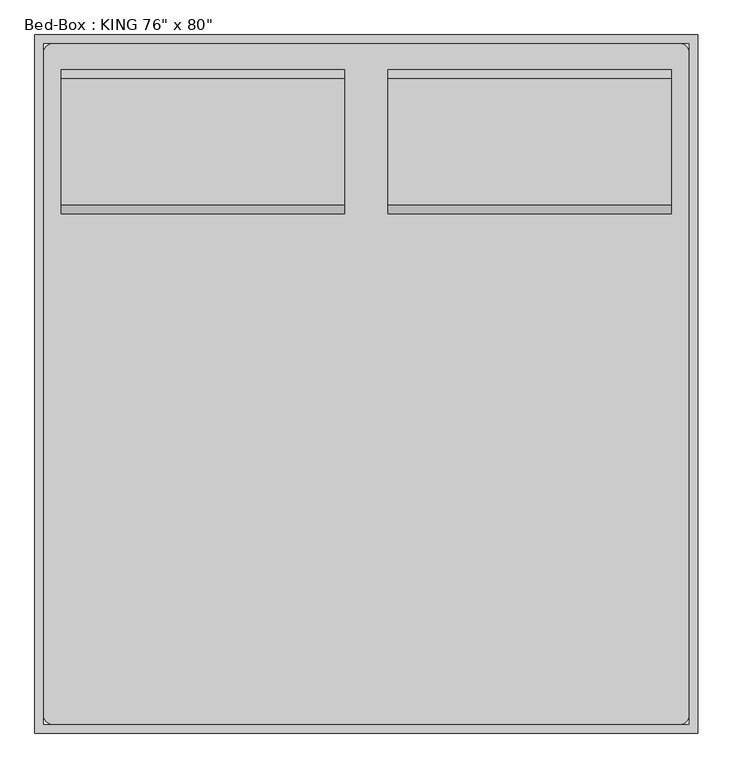
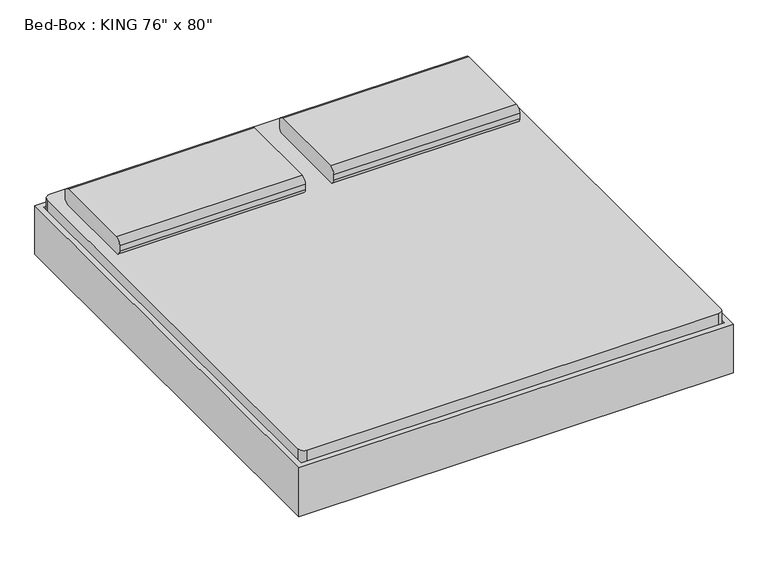
"""IFC4 building model written with IfcOpenShell, lengths in millimetres: furniture geometry."""

from ifc_helpers import new_model, si_unit, point, frame, frame_2d, origin, place, context, project, spatial, polyline, circle_curve, trimmed, segment, composite_curve, outline, extrude, source, transform, mapped, element, save
from ifc_brep_helpers import plane_surface, cylinder_surface, revolved_surface, advanced_brep


def furniture_3daafeb3(model_context):
    return source(origin(), model_context, "Body", "SolidModel", [
        extrude(outline(composite_curve([segment(polyline([(654.5704918, 406.4), (286.2704918, 406.4)]), True, "CONTINUOUS"), segment(trimmed(circle_curve(frame_2d((286.2704918, 431.8)), 25.4), [point((286.2704918, 406.4))], [point((260.8704918, 431.8))], False, "CARTESIAN"), True, "CONTINUOUS"), segment(polyline([(260.8704918, 431.8), (260.8704918, 457.2)]), True, "CONTINUOUS"), segment(trimmed(circle_curve(frame_2d((286.2704918, 457.2)), 25.4), [point((260.8704918, 457.2))], [point((286.2704918, 482.6))], False, "CARTESIAN"), True, "CONTINUOUS"), segment(polyline([(286.2704918, 482.6), (654.5704918, 482.6)]), True, "CONTINUOUS"), segment(trimmed(circle_curve(frame_2d((654.5704918, 457.2)), 25.4), [point((654.5704918, 482.6))], [point((679.9704918, 457.2))], False, "CARTESIAN"), True, "CONTINUOUS"), segment(polyline([(679.9704918, 457.2), (679.9704918, 431.8)]), True, "CONTINUOUS"), segment(trimmed(circle_curve(frame_2d((654.5704918, 431.8)), 25.4), [point((679.9704918, 431.8))], [point((654.5704918, 406.4))], False, "CARTESIAN"), True, "CONTINUOUS")], self_intersect=False)), frame((402.652459, 0.0, 0.0), z_axis=(1.0, 0.0, 0.0), x_axis=(0.0, 1.0, 0.0)), (0.0, 0.0, 1.0), 825.5),
        extrude(outline(composite_curve([segment(polyline([(654.5704918, 406.4), (286.2704918, 406.4)]), True, "CONTINUOUS"), segment(trimmed(circle_curve(frame_2d((286.2704918, 431.8)), 25.4), [point((286.2704918, 406.4))], [point((260.8704918, 431.8))], False, "CARTESIAN"), True, "CONTINUOUS"), segment(polyline([(260.8704918, 431.8), (260.8704918, 457.2)]), True, "CONTINUOUS"), segment(trimmed(circle_curve(frame_2d((286.2704918, 457.2)), 25.4), [point((260.8704918, 457.2))], [point((286.2704918, 482.6))], False, "CARTESIAN"), True, "CONTINUOUS"), segment(polyline([(286.2704918, 482.6), (654.5704918, 482.6)]), True, "CONTINUOUS"), segment(trimmed(circle_curve(frame_2d((654.5704918, 457.2)), 25.4), [point((654.5704918, 482.6))], [point((679.9704918, 457.2))], False, "CARTESIAN"), True, "CONTINUOUS"), segment(polyline([(679.9704918, 457.2), (679.9704918, 431.8)]), True, "CONTINUOUS"), segment(trimmed(circle_curve(frame_2d((654.5704918, 431.8)), 25.4), [point((679.9704918, 431.8))], [point((654.5704918, 406.4))], False, "CARTESIAN"), True, "CONTINUOUS")], self_intersect=False)), frame((-549.847541, 0.0, 0.0), z_axis=(1.0, 0.0, 0.0), x_axis=(0.0, 1.0, 0.0)), (0.0, 0.0, 1.0), 825.5),
        advanced_brep(
        [(-600.3231784, 527.5704918, 177.8), (-600.3231784, 451.3704918, 177.8), (-600.3231784, 451.3704918, 196.85), (-600.3231784, 527.5704918, 196.85), (-549.5231784, 527.5704918, 177.8), (-549.5231784, 451.3704918, 177.8), (-537.3869899, 451.3704918, 196.85), (-537.3869899, 527.5704918, 196.85), (-473.4523099, 527.5704918, 14.6654962), (-473.4523099, 451.3704918, 14.6654962), (-456.1871466, 451.3704918, 22.716374), (-456.1871466, 527.5704918, 22.716374), (-450.4320921, 451.3704918, 0.0), (-450.4320921, 527.5704918, 0.0), (-450.4320921, 451.3704918, 19.05), (-450.4320921, 527.5704918, 19.05), (-371.8195862, 527.5704918, 0.0), (-371.8195862, 451.3704918, 0.0), (-371.8195862, 451.3704918, 19.05), (-371.8195862, 527.5704918, 19.05), (-359.1195862, 451.3704918, 3.4029547), (-359.1195862, 527.5704918, 3.4029547), (-368.6445862, 451.3704918, 19.9007387), (-368.6445862, 527.5704918, 19.9007387), (-299.022541, 527.5704918, 38.1), (-299.022541, 451.3704918, 38.1), (-304.1269731, 451.3704918, 57.15), (-304.1269731, 527.5704918, 57.15), (977.6518216, 527.5704918, 38.1), (977.6518216, 451.3704918, 38.1), (982.7562537, 451.3704918, 57.15), (982.7562537, 527.5704918, 57.15), (1037.7488669, 527.5704918, 3.4029547), (1037.7488669, 451.3704918, 3.4029547), (1047.2738669, 451.3704918, 19.9007387), (1047.2738669, 527.5704918, 19.9007387), (1050.4488669, 451.3704918, 0.0), (1050.4488669, 527.5704918, 0.0), (1050.4488669, 451.3704918, 19.05), (1050.4488669, 527.5704918, 19.05), (1129.0613728, 527.5704918, 0.0), (1129.0613728, 451.3704918, 0.0), (1129.0613728, 451.3704918, 19.05), (1129.0613728, 527.5704918, 19.05), (1152.0815906, 451.3704918, 14.6654962), (1152.0815906, 527.5704918, 14.6654962), (1134.8164272, 451.3704918, 22.716374), (1134.8164272, 527.5704918, 22.716374), (1228.152459, 527.5704918, 177.8), (1228.152459, 451.3704918, 177.8), (1216.0162705, 451.3704918, 196.85), (1216.0162705, 527.5704918, 196.85), (1278.952459, 527.5704918, 177.8), (1278.952459, 527.5704918, 196.85), (1278.952459, 451.3704918, 196.85), (1278.952459, 451.3704918, 177.8)],
        [
            (0, 1),
            (1, 2),
            (2, 3),
            (3, 0),
            (0, 4),
            (4, 5),
            (5, 1),
            (5, 6),
            (6, 2),
            (6, 7),
            (7, 3),
            (7, 4),
            (4, 8),
            (8, 9),
            (9, 5),
            (9, 10),
            (10, 6),
            (10, 11),
            (11, 7),
            (11, 8),
            (12, 9, circle_curve(frame((-450.4320921, 451.3704918, 25.4), z_axis=(0.0, 1.0, 0.0), x_axis=(-0.9063077870366486, 0.0, -0.42261826174070233)), 25.4)),
            (8, 13, circle_curve(frame((-450.4320921, 527.5704918, 25.4), z_axis=(0.0, -1.0, 0.0), x_axis=(-0.9063077870366486, 0.0, -0.42261826174070233)), 25.4)),
            (13, 12),
            (14, 10, circle_curve(frame((-450.4320921, 451.3704918, 25.4), z_axis=(0.0, 1.0, 0.0), x_axis=(-0.9063077870366486, 0.0, -0.42261826174070233)), 6.35)),
            (12, 14),
            (15, 11, circle_curve(frame((-450.4320921, 527.5704918, 25.4), z_axis=(0.0, 1.0, 0.0), x_axis=(-0.9063077870366486, 0.0, -0.42261826174070233)), 6.35)),
            (14, 15),
            (15, 13),
            (13, 16),
            (16, 17),
            (17, 12),
            (17, 18),
            (18, 14),
            (18, 19),
            (19, 15),
            (19, 16),
            (20, 17, circle_curve(frame((-371.8195862, 451.3704918, 25.4), z_axis=(0.0, 1.0, 0.0), x_axis=(0.0, 0.0, -1.0)), 25.4)),
            (16, 21, circle_curve(frame((-371.8195862, 527.5704918, 25.4), z_axis=(0.0, -1.0, 0.0), x_axis=(0.0, 0.0, -1.0)), 25.4)),
            (21, 20),
            (22, 18, circle_curve(frame((-371.8195862, 451.3704918, 25.4), z_axis=(0.0, 1.0, 0.0), x_axis=(0.0, 0.0, -1.0)), 6.35)),
            (20, 22),
            (23, 19, circle_curve(frame((-371.8195862, 527.5704918, 25.4), z_axis=(0.0, 1.0, 0.0), x_axis=(0.0, 0.0, -1.0)), 6.35)),
            (22, 23),
            (23, 21),
            (21, 24),
            (24, 25),
            (25, 20),
            (25, 26),
            (26, 22),
            (26, 27),
            (27, 23),
            (27, 24),
            (24, 28),
            (28, 29),
            (29, 25),
            (29, 30),
            (30, 26),
            (30, 31),
            (31, 27),
            (31, 28),
            (28, 32),
            (32, 33),
            (33, 29),
            (33, 34),
            (34, 30),
            (34, 35),
            (35, 31),
            (35, 32),
            (36, 33, circle_curve(frame((1050.4488669, 451.3704918, 25.4), z_axis=(0.0, 1.0, 0.0), x_axis=(-0.5000000000000463, 0.0, -0.8660254037844118)), 25.4)),
            (32, 37, circle_curve(frame((1050.4488669, 527.5704918, 25.4), z_axis=(0.0, -1.0, 0.0), x_axis=(-0.5000000000000463, 0.0, -0.8660254037844118)), 25.4)),
            (37, 36),
            (38, 34, circle_curve(frame((1050.4488669, 451.3704918, 25.4), z_axis=(0.0, 1.0, 0.0), x_axis=(-0.5000000000000463, 0.0, -0.8660254037844118)), 6.35)),
            (36, 38),
            (39, 35, circle_curve(frame((1050.4488669, 527.5704918, 25.4), z_axis=(0.0, 1.0, 0.0), x_axis=(-0.5000000000000463, 0.0, -0.8660254037844118)), 6.35)),
            (38, 39),
            (39, 37),
            (37, 40),
            (40, 41),
            (41, 36),
            (41, 42),
            (42, 38),
            (42, 43),
            (43, 39),
            (43, 40),
            (44, 41, circle_curve(frame((1129.0613728, 451.3704918, 25.4), z_axis=(0.0, 1.0, 0.0), x_axis=(0.0, 0.0, -1.0)), 25.4)),
            (40, 45, circle_curve(frame((1129.0613728, 527.5704918, 25.4), z_axis=(0.0, -1.0, 0.0), x_axis=(0.0, 0.0, -1.0)), 25.4)),
            (45, 44),
            (46, 42, circle_curve(frame((1129.0613728, 451.3704918, 25.4), z_axis=(0.0, 1.0, 0.0), x_axis=(0.0, 0.0, -1.0)), 6.35)),
            (44, 46),
            (47, 43, circle_curve(frame((1129.0613728, 527.5704918, 25.4), z_axis=(0.0, 1.0, 0.0), x_axis=(0.0, 0.0, -1.0)), 6.35)),
            (46, 47),
            (47, 45),
            (45, 48),
            (48, 49),
            (49, 44),
            (49, 50),
            (50, 46),
            (50, 51),
            (51, 47),
            (51, 48),
            (52, 53),
            (53, 54),
            (54, 55),
            (55, 52),
            (48, 52),
            (55, 49),
            (54, 50),
            (53, 51),
        ],
        [
            plane_surface(frame((-600.3231784, 781.5704918, -152.9490627), z_axis=(-1.0, 0.0, 0.0), x_axis=(0.0, 1.0, 0.0))),
            plane_surface(frame((-600.3231784, 527.5704918, 177.8), z_axis=(0.0, 0.0, -1.0), x_axis=(1.0, 0.0, 0.0))),
            plane_surface(frame((-600.3231784, 451.3704918, 177.8), z_axis=(0.0, -1.0, 0.0), x_axis=(1.0, 0.0, 0.0))),
            plane_surface(frame((-600.3231784, 451.3704918, 196.85), z_axis=(0.0, 0.0, 1.0), x_axis=(1.0, 0.0, 0.0))),
            plane_surface(frame((-600.3231784, 527.5704918, 196.85), z_axis=(0.0, 1.0, 0.0), x_axis=(1.0, 0.0, 0.0))),
            plane_surface(frame((-549.5231784, 527.5704918, 177.8), z_axis=(-0.9063077870366487, 0.0, -0.4226182617407022), x_axis=(0.4226182617407022, 0.0, -0.9063077870366487))),
            plane_surface(frame((-549.5231784, 451.3704918, 177.8), z_axis=(0.0, -1.0, 0.0), x_axis=(0.42261826174070183, 0.0, -0.9063077870366488))),
            plane_surface(frame((-537.3869899, 451.3704918, 196.85), z_axis=(0.9063077870366485, 0.0, 0.42261826174070277), x_axis=(0.42261826174070277, 0.0, -0.9063077870366485))),
            plane_surface(frame((-537.3869899, 527.5704918, 196.85), z_axis=(0.0, 1.0000000000000002, 0.0), x_axis=(0.4226182617407021, 0.0, -0.9063077870366487))),
            cylinder_surface(frame((-450.4320921, 781.5704918, 25.4), z_axis=(0.0, -1.0, 0.0), x_axis=(-0.9063077870366486, 0.0, -0.42261826174070233)), 25.4),
            plane_surface(frame((-450.4320921, 451.3704918, 25.4), z_axis=(0.0, -1.0, 0.0), x_axis=(-0.9063077870366486, 0.0, -0.42261826174070233))),
            revolved_surface(polyline([(-456.1871465476827, 451.3704918, 22.71637403794654), (-456.1871465476827, 527.5704918, 22.71637403794654)]), (-450.4320921, 781.5704918, 25.4), (0.0, -1.0, 0.0)),
            plane_surface(frame((-450.4320921, 527.5704918, 25.4), z_axis=(0.0, 1.0, 0.0), x_axis=(-0.9063077870366486, 0.0, -0.42261826174070233))),
            plane_surface(frame((-450.4320921, 527.5704918, 0.0), z_axis=(0.0, 0.0, -1.0), x_axis=(1.0, 0.0, 0.0))),
            plane_surface(frame((-450.4320921, 451.3704918, 0.0), z_axis=(0.0, -1.0, 0.0), x_axis=(1.0, 0.0, 0.0))),
            plane_surface(frame((-450.4320921, 451.3704918, 19.05), z_axis=(0.0, 0.0, 1.0), x_axis=(1.0, 0.0, 0.0))),
            plane_surface(frame((-450.4320921, 527.5704918, 19.05), z_axis=(0.0, 1.0, 0.0), x_axis=(1.0, 0.0, 0.0))),
            cylinder_surface(frame((-371.8195862, 781.5704918, 25.4), z_axis=(0.0, -1.0, 0.0), x_axis=(0.0, 0.0, -1.0)), 25.4),
            plane_surface(frame((-371.8195862, 451.3704918, 25.4), z_axis=(0.0, -1.0, 0.0), x_axis=(0.0, 0.0, -1.0))),
            revolved_surface(polyline([(-371.8195862, 451.3704918, 19.049999999999997), (-371.8195862, 527.5704918, 19.049999999999997)]), (-371.8195862, 781.5704918, 25.4), (0.0, -1.0, 0.0)),
            plane_surface(frame((-371.8195862, 527.5704918, 25.4), z_axis=(0.0, 1.0, 0.0), x_axis=(0.0, 0.0, -1.0))),
            plane_surface(frame((-359.1195862, 527.5704918, 3.4029547), z_axis=(0.4999999999998777, 0.0, -0.8660254037845092), x_axis=(0.8660254037845092, 0.0, 0.4999999999998777))),
            plane_surface(frame((-359.1195862, 451.3704918, 3.4029547), z_axis=(0.0, -1.0, 0.0), x_axis=(0.8660254037845095, 0.0, 0.49999999999987715))),
            plane_surface(frame((-368.6445862, 451.3704918, 19.9007387), z_axis=(-0.49999999999987793, 0.0, 0.8660254037845091), x_axis=(0.8660254037845091, 0.0, 0.49999999999987793))),
            plane_surface(frame((-368.6445862, 527.5704918, 19.9007387), z_axis=(0.0, 1.0, 0.0), x_axis=(0.8660254037845092, 0.0, 0.49999999999987776))),
            plane_surface(frame((-299.022541, 527.5704918, 38.1), z_axis=(0.0, 0.0, -1.0), x_axis=(1.0, 0.0, 0.0))),
            plane_surface(frame((-299.022541, 451.3704918, 38.1), z_axis=(0.0, -1.0, 0.0), x_axis=(1.0, 0.0, 0.0))),
            plane_surface(frame((-304.1269731, 451.3704918, 57.15), z_axis=(0.0, 0.0, 1.0), x_axis=(1.0, 0.0, 0.0))),
            plane_surface(frame((-304.1269731, 527.5704918, 57.15), z_axis=(0.0, 1.0, 0.0), x_axis=(1.0, 0.0, 0.0))),
            plane_surface(frame((977.6518216, 527.5704918, 38.1), z_axis=(-0.5000000000000457, 0.0, -0.8660254037844123), x_axis=(0.8660254037844123, 0.0, -0.5000000000000457))),
            plane_surface(frame((977.6518216, 451.3704918, 38.1), z_axis=(0.0, -1.0000000000000002, 0.0), x_axis=(0.866025403784412, 0.0, -0.5000000000000464))),
            plane_surface(frame((982.7562537, 451.3704918, 57.15), z_axis=(0.5000000000000454, 0.0, 0.8660254037844125), x_axis=(0.8660254037844125, 0.0, -0.5000000000000454))),
            plane_surface(frame((982.7562537, 527.5704918, 57.15), z_axis=(0.0, 1.0, 0.0), x_axis=(0.8660254037844126, 0.0, -0.5000000000000452))),
            cylinder_surface(frame((1050.4488669, 781.5704918, 25.4), z_axis=(0.0, -1.0, 0.0), x_axis=(-0.5000000000000463, 0.0, -0.8660254037844118)), 25.4),
            plane_surface(frame((1050.4488669, 451.3704918, 25.4), z_axis=(0.0, -1.0000000000000002, 0.0), x_axis=(-0.5000000000000464, 0.0, -0.866025403784412))),
            revolved_surface(polyline([(1047.2738668999998, 451.3704918, 19.90073868596898), (1047.2738668999998, 527.5704918, 19.90073868596898)]), (1050.4488669, 781.5704918, 25.4), (0.0, -1.0, 0.0)),
            plane_surface(frame((1050.4488669, 527.5704918, 25.4), z_axis=(0.0, 1.0000000000000002, 0.0), x_axis=(-0.5000000000000464, 0.0, -0.866025403784412))),
            plane_surface(frame((1050.4488669, 527.5704918, 0.0), z_axis=(0.0, 0.0, -1.0), x_axis=(1.0, 0.0, 0.0))),
            plane_surface(frame((1050.4488669, 451.3704918, 0.0), z_axis=(0.0, -1.0, 0.0), x_axis=(1.0, 0.0, 0.0))),
            plane_surface(frame((1050.4488669, 451.3704918, 19.05), z_axis=(0.0, 0.0, 1.0), x_axis=(1.0, 0.0, 0.0))),
            plane_surface(frame((1050.4488669, 527.5704918, 19.05), z_axis=(0.0, 1.0, 0.0), x_axis=(1.0, 0.0, 0.0))),
            cylinder_surface(frame((1129.0613728, 781.5704918, 25.4), z_axis=(0.0, -1.0, 0.0), x_axis=(0.0, 0.0, -1.0)), 25.4),
            plane_surface(frame((1129.0613728, 451.3704918, 25.4), z_axis=(0.0, -1.0, 0.0), x_axis=(0.0, 0.0, -1.0))),
            revolved_surface(polyline([(1129.0613728, 451.3704918, 19.049999999999997), (1129.0613728, 527.5704918, 19.049999999999997)]), (1129.0613728, 781.5704918, 25.4), (0.0, -1.0, 0.0)),
            plane_surface(frame((1129.0613728, 527.5704918, 25.4), z_axis=(0.0, 1.0, 0.0), x_axis=(0.0, 0.0, -1.0))),
            plane_surface(frame((1152.0815906, 527.5704918, 14.6654962), z_axis=(0.9063077870366798, 0.0, -0.42261826174063555), x_axis=(0.42261826174063555, 0.0, 0.9063077870366798))),
            plane_surface(frame((1152.0815906, 451.3704918, 14.6654962), z_axis=(0.0, -1.0, 0.0), x_axis=(0.4226182617406357, 0.0, 0.9063077870366797))),
            plane_surface(frame((1134.8164272, 451.3704918, 22.716374), z_axis=(-0.9063077870366798, 0.0, 0.4226182617406355), x_axis=(0.4226182617406355, 0.0, 0.9063077870366798))),
            plane_surface(frame((1134.8164272, 527.5704918, 22.716374), z_axis=(0.0, 1.0000000000000002, 0.0), x_axis=(0.4226182617406361, 0.0, 0.9063077870366796))),
            plane_surface(frame((1278.952459, 781.5704918, -152.9490627), z_axis=(1.0, 0.0, 0.0), x_axis=(0.0, 1.0, 0.0))),
            plane_surface(frame((1228.152459, 527.5704918, 177.8), z_axis=(0.0, 0.0, -1.0), x_axis=(1.0, 0.0, 0.0))),
            plane_surface(frame((1228.152459, 451.3704918, 177.8), z_axis=(0.0, -1.0, 0.0), x_axis=(1.0, 0.0, 0.0))),
            plane_surface(frame((1216.0162705, 451.3704918, 196.85), z_axis=(0.0, 0.0, 1.0), x_axis=(1.0, 0.0, 0.0))),
            plane_surface(frame((1216.0162705, 527.5704918, 196.85), z_axis=(0.0, 1.0, 0.0), x_axis=(1.0, 0.0, 0.0))),
        ],
        [
            (0, [[1, 2, 3, 4]]),
            (1, [[-1, 5, 6, 7]]),
            (2, [[-2, -7, 8, 9]]),
            (3, [[-3, -9, 10, 11]]),
            (4, [[-4, -11, 12, -5]]),
            (5, [[-6, 13, 14, 15]]),
            (6, [[-8, -15, 16, 17]]),
            (7, [[-10, -17, 18, 19]]),
            (8, [[-12, -19, 20, -13]]),
            (9, [[21, -14, 22, 23]]),
            (10, [[24, -16, -21, 25]]),
            (11, [[26, -18, -24, 27]]),
            (12, [[-22, -20, -26, 28]]),
            (13, [[-23, 29, 30, 31]]),
            (14, [[-25, -31, 32, 33]]),
            (15, [[-27, -33, 34, 35]]),
            (16, [[-28, -35, 36, -29]]),
            (17, [[37, -30, 38, 39]]),
            (18, [[40, -32, -37, 41]]),
            (19, [[42, -34, -40, 43]]),
            (20, [[-38, -36, -42, 44]]),
            (21, [[-39, 45, 46, 47]]),
            (22, [[-41, -47, 48, 49]]),
            (23, [[-43, -49, 50, 51]]),
            (24, [[-44, -51, 52, -45]]),
            (25, [[-46, 53, 54, 55]]),
            (26, [[-48, -55, 56, 57]]),
            (27, [[-50, -57, 58, 59]]),
            (28, [[-52, -59, 60, -53]]),
            (29, [[-54, 61, 62, 63]]),
            (30, [[-56, -63, 64, 65]]),
            (31, [[-58, -65, 66, 67]]),
            (32, [[-60, -67, 68, -61]]),
            (33, [[69, -62, 70, 71]]),
            (34, [[72, -64, -69, 73]]),
            (35, [[74, -66, -72, 75]]),
            (36, [[-70, -68, -74, 76]]),
            (37, [[-71, 77, 78, 79]]),
            (38, [[-73, -79, 80, 81]]),
            (39, [[-75, -81, 82, 83]]),
            (40, [[-76, -83, 84, -77]]),
            (41, [[85, -78, 86, 87]]),
            (42, [[88, -80, -85, 89]]),
            (43, [[90, -82, -88, 91]]),
            (44, [[-86, -84, -90, 92]]),
            (45, [[-87, 93, 94, 95]]),
            (46, [[-89, -95, 96, 97]]),
            (47, [[-91, -97, 98, 99]]),
            (48, [[-92, -99, 100, -93]]),
            (49, [[101, 102, 103, 104]]),
            (50, [[-94, 105, -104, 106]]),
            (51, [[-96, -106, -103, 107]]),
            (52, [[-98, -107, -102, 108]]),
            (53, [[-100, -108, -101, -105]]),
        ],
    ),
        extrude(outline(composite_curve([segment(polyline([(-575.247541, 756.1704918), (1253.552459, 756.1704918)]), True, "CONTINUOUS"), segment(trimmed(circle_curve(frame_2d((1253.552459, 730.7704918)), 25.4), [point((1253.552459, 756.1704918))], [point((1278.952459, 730.7704918))], False, "CARTESIAN"), True, "CONTINUOUS"), segment(polyline([(1278.952459, 730.7704918), (1278.952459, -1199.6295082)]), True, "CONTINUOUS"), segment(trimmed(circle_curve(frame_2d((1253.552459, -1199.6295082)), 25.4), [point((1278.952459, -1199.6295082))], [point((1253.552459, -1225.0295082))], False, "CARTESIAN"), True, "CONTINUOUS"), segment(polyline([(1253.552459, -1225.0295082), (-575.247541, -1225.0295082)]), True, "CONTINUOUS"), segment(trimmed(circle_curve(frame_2d((-575.247541, -1199.6295082)), 25.4), [point((-575.247541, -1225.0295082))], [point((-600.647541, -1199.6295082))], False, "CARTESIAN"), True, "CONTINUOUS"), segment(polyline([(-600.647541, -1199.6295082), (-600.647541, 730.7704918)]), True, "CONTINUOUS"), segment(trimmed(circle_curve(frame_2d((-575.247541, 730.7704918)), 25.4), [point((-600.647541, 730.7704918))], [point((-575.247541, 756.1704918))], False, "CARTESIAN"), True, "CONTINUOUS")], self_intersect=False)), frame((0.0, 0.0, 203.2), z_axis=(0.0, 0.0, 1.0), x_axis=(1.0, 0.0, 0.0)), (0.0, 0.0, 1.0), 203.2),
        advanced_brep(
        [(-600.647541, -945.6295082, 196.85), (-600.647541, -945.6295082, 177.8), (-600.647541, -1021.8295082, 177.8), (-600.647541, -1021.8295082, 196.85), (-537.7113525, -945.6295082, 196.85), (-549.847541, -945.6295082, 177.8), (-549.847541, -1021.8295082, 177.8), (-537.7113525, -1021.8295082, 196.85), (-456.5115092, -945.6295082, 22.716374), (-473.7766725, -945.6295082, 14.6654962), (-473.7766725, -1021.8295082, 14.6654962), (-456.5115092, -1021.8295082, 22.716374), (-450.7564547, -945.6295082, 0.0), (-450.7564547, -945.6295082, 19.05), (-450.7564547, -1021.8295082, 0.0), (-450.7564547, -1021.8295082, 19.05), (-372.1439489, -945.6295082, 19.05), (-372.1439489, -945.6295082, 0.0), (-372.1439489, -1021.8295082, 0.0), (-372.1439489, -1021.8295082, 19.05), (-359.4439489, -945.6295082, 3.4029547), (-368.9689489, -945.6295082, 19.9007387), (-359.4439489, -1021.8295082, 3.4029547), (-368.9689489, -1021.8295082, 19.9007387), (-304.4513357, -945.6295082, 57.15), (-299.3469036, -945.6295082, 38.1), (-299.3469036, -1021.8295082, 38.1), (-304.4513357, -1021.8295082, 57.15), (982.7562537, -945.6295082, 57.15), (977.6518216, -945.6295082, 38.1), (977.6518216, -1021.8295082, 38.1), (982.7562537, -1021.8295082, 57.15), (1047.2738669, -945.6295082, 19.9007387), (1037.7488669, -945.6295082, 3.4029547), (1037.7488669, -1021.8295082, 3.4029547), (1047.2738669, -1021.8295082, 19.9007387), (1050.4488669, -945.6295082, 0.0), (1050.4488669, -945.6295082, 19.05), (1050.4488669, -1021.8295082, 0.0), (1050.4488669, -1021.8295082, 19.05), (1129.0613728, -945.6295082, 19.05), (1129.0613728, -945.6295082, 0.0), (1129.0613728, -1021.8295082, 0.0), (1129.0613728, -1021.8295082, 19.05), (1152.0815906, -945.6295082, 14.6654962), (1134.8164272, -945.6295082, 22.716374), (1152.0815906, -1021.8295082, 14.6654962), (1134.8164272, -1021.8295082, 22.716374), (1216.0162705, -945.6295082, 196.85), (1228.152459, -945.6295082, 177.8), (1228.152459, -1021.8295082, 177.8), (1216.0162705, -1021.8295082, 196.85), (1278.952459, -945.6295082, 196.85), (1278.952459, -1021.8295082, 196.85), (1278.952459, -1021.8295082, 177.8), (1278.952459, -945.6295082, 177.8)],
        [
            (0, 1),
            (1, 2),
            (2, 3),
            (3, 0),
            (0, 4),
            (4, 5),
            (5, 1),
            (5, 6),
            (6, 2),
            (6, 7),
            (7, 3),
            (7, 4),
            (4, 8),
            (8, 9),
            (9, 5),
            (9, 10),
            (10, 6),
            (10, 11),
            (11, 7),
            (11, 8),
            (12, 9, circle_curve(frame((-450.7564547, -945.6295082, 25.4), z_axis=(0.0, 1.0, 0.0), x_axis=(-0.906307787036663, 0.0, -0.4226182617406713)), 25.4)),
            (8, 13, circle_curve(frame((-450.7564547, -945.6295082, 25.4), z_axis=(0.0, -1.0, 0.0), x_axis=(-0.906307787036663, 0.0, -0.4226182617406713)), 6.35)),
            (13, 12),
            (14, 10, circle_curve(frame((-450.7564547, -1021.8295082, 25.4), z_axis=(0.0, 1.0, 0.0), x_axis=(-0.906307787036663, 0.0, -0.4226182617406713)), 25.4)),
            (12, 14),
            (15, 11, circle_curve(frame((-450.7564547, -1021.8295082, 25.4), z_axis=(0.0, 1.0, 0.0), x_axis=(-0.906307787036663, 0.0, -0.4226182617406713)), 6.35)),
            (14, 15),
            (15, 13),
            (13, 16),
            (16, 17),
            (17, 12),
            (17, 18),
            (18, 14),
            (18, 19),
            (19, 15),
            (19, 16),
            (20, 17, circle_curve(frame((-372.1439489, -945.6295082, 25.4), z_axis=(0.0, 1.0, 0.0), x_axis=(0.0, 0.0, -1.0)), 25.4)),
            (16, 21, circle_curve(frame((-372.1439489, -945.6295082, 25.4), z_axis=(0.0, -1.0, 0.0), x_axis=(0.0, 0.0, -1.0)), 6.35)),
            (21, 20),
            (22, 18, circle_curve(frame((-372.1439489, -1021.8295082, 25.4), z_axis=(0.0, 1.0, 0.0), x_axis=(0.0, 0.0, -1.0)), 25.4)),
            (20, 22),
            (23, 19, circle_curve(frame((-372.1439489, -1021.8295082, 25.4), z_axis=(0.0, 1.0, 0.0), x_axis=(0.0, 0.0, -1.0)), 6.35)),
            (22, 23),
            (23, 21),
            (21, 24),
            (24, 25),
            (25, 20),
            (25, 26),
            (26, 22),
            (26, 27),
            (27, 23),
            (27, 24),
            (24, 28),
            (28, 29),
            (29, 25),
            (29, 30),
            (30, 26),
            (30, 31),
            (31, 27),
            (31, 28),
            (28, 32),
            (32, 33),
            (33, 29),
            (33, 34),
            (34, 30),
            (34, 35),
            (35, 31),
            (35, 32),
            (36, 33, circle_curve(frame((1050.4488669, -945.6295082, 25.4), z_axis=(0.0, 1.0, 0.0), x_axis=(-0.5000000000000479, 0.0, -0.866025403784411)), 25.4)),
            (32, 37, circle_curve(frame((1050.4488669, -945.6295082, 25.4), z_axis=(0.0, -1.0, 0.0), x_axis=(-0.5000000000000479, 0.0, -0.866025403784411)), 6.35)),
            (37, 36),
            (38, 34, circle_curve(frame((1050.4488669, -1021.8295082, 25.4), z_axis=(0.0, 1.0, 0.0), x_axis=(-0.5000000000000479, 0.0, -0.866025403784411)), 25.4)),
            (36, 38),
            (39, 35, circle_curve(frame((1050.4488669, -1021.8295082, 25.4), z_axis=(0.0, 1.0, 0.0), x_axis=(-0.5000000000000479, 0.0, -0.866025403784411)), 6.35)),
            (38, 39),
            (39, 37),
            (37, 40),
            (40, 41),
            (41, 36),
            (41, 42),
            (42, 38),
            (42, 43),
            (43, 39),
            (43, 40),
            (44, 41, circle_curve(frame((1129.0613728, -945.6295082, 25.4), z_axis=(0.0, 1.0, 0.0), x_axis=(0.0, 0.0, -1.0)), 25.4)),
            (40, 45, circle_curve(frame((1129.0613728, -945.6295082, 25.4), z_axis=(0.0, -1.0, 0.0), x_axis=(0.0, 0.0, -1.0)), 6.35)),
            (45, 44),
            (46, 42, circle_curve(frame((1129.0613728, -1021.8295082, 25.4), z_axis=(0.0, 1.0, 0.0), x_axis=(0.0, 0.0, -1.0)), 25.4)),
            (44, 46),
            (47, 43, circle_curve(frame((1129.0613728, -1021.8295082, 25.4), z_axis=(0.0, 1.0, 0.0), x_axis=(0.0, 0.0, -1.0)), 6.35)),
            (46, 47),
            (47, 45),
            (45, 48),
            (48, 49),
            (49, 44),
            (49, 50),
            (50, 46),
            (50, 51),
            (51, 47),
            (51, 48),
            (52, 53),
            (53, 54),
            (54, 55),
            (55, 52),
            (48, 52),
            (55, 49),
            (54, 50),
            (53, 51),
        ],
        [
            plane_surface(frame((-600.647541, -1250.4295082, -127.5947323), z_axis=(-1.0, 0.0, 0.0), x_axis=(0.0, 1.0, 0.0))),
            plane_surface(frame((-600.647541, -945.6295082, 196.85), z_axis=(0.0, 1.0, 0.0), x_axis=(1.0, 0.0, 0.0))),
            plane_surface(frame((-600.647541, -945.6295082, 177.8), z_axis=(0.0, 0.0, -1.0), x_axis=(1.0, 0.0, 0.0))),
            plane_surface(frame((-600.647541, -1021.8295082, 177.8), z_axis=(0.0, -1.0, 0.0), x_axis=(1.0, 0.0, 0.0))),
            plane_surface(frame((-600.647541, -1021.8295082, 196.85), z_axis=(0.0, 0.0, 1.0), x_axis=(1.0, 0.0, 0.0))),
            plane_surface(frame((-537.7113525, -945.6295082, 196.85), z_axis=(0.0, 1.0, 0.0), x_axis=(0.422618261740671, 0.0, -0.9063077870366633))),
            plane_surface(frame((-549.847541, -945.6295082, 177.8), z_axis=(-0.9063077870366631, 0.0, -0.42261826174067135), x_axis=(0.42261826174067135, 0.0, -0.9063077870366631))),
            plane_surface(frame((-549.847541, -1021.8295082, 177.8), z_axis=(0.0, -1.0, 0.0), x_axis=(0.42261826174067124, 0.0, -0.9063077870366631))),
            plane_surface(frame((-537.7113525, -1021.8295082, 196.85), z_axis=(0.9063077870366631, 0.0, 0.4226182617406712), x_axis=(0.4226182617406712, 0.0, -0.9063077870366631))),
            plane_surface(frame((-450.7564547, -945.6295082, 25.4), z_axis=(0.0, 1.0, 0.0), x_axis=(-0.906307787036663, 0.0, -0.4226182617406713))),
            cylinder_surface(frame((-450.7564547, -1250.4295082, 25.4), z_axis=(0.0, -1.0, 0.0), x_axis=(-0.906307787036663, 0.0, -0.4226182617406713)), 25.4),
            plane_surface(frame((-450.7564547, -1021.8295082, 25.4), z_axis=(0.0, -1.0, 0.0), x_axis=(-0.906307787036663, 0.0, -0.4226182617406713))),
            revolved_surface(polyline([(-456.51150914768283, -1021.8295082, 22.716374037946736), (-456.51150914768283, -945.6295082, 22.716374037946736)]), (-450.7564547, -1250.4295082, 25.4), (0.0, -1.0, 0.0)),
            plane_surface(frame((-450.7564547, -945.6295082, 19.05), z_axis=(0.0, 1.0, 0.0), x_axis=(1.0, 0.0, 0.0))),
            plane_surface(frame((-450.7564547, -945.6295082, 0.0), z_axis=(0.0, 0.0, -1.0), x_axis=(1.0, 0.0, 0.0))),
            plane_surface(frame((-450.7564547, -1021.8295082, 0.0), z_axis=(0.0, -1.0, 0.0), x_axis=(1.0, 0.0, 0.0))),
            plane_surface(frame((-450.7564547, -1021.8295082, 19.05), z_axis=(0.0, 0.0, 1.0), x_axis=(1.0, 0.0, 0.0))),
            plane_surface(frame((-372.1439489, -945.6295082, 25.4), z_axis=(0.0, 1.0, 0.0), x_axis=(0.0, 0.0, -1.0))),
            cylinder_surface(frame((-372.1439489, -1250.4295082, 25.4), z_axis=(0.0, -1.0, 0.0), x_axis=(0.0, 0.0, -1.0)), 25.4),
            plane_surface(frame((-372.1439489, -1021.8295082, 25.4), z_axis=(0.0, -1.0, 0.0), x_axis=(0.0, 0.0, -1.0))),
            revolved_surface(polyline([(-372.1439489, -1021.8295082, 19.049999999999997), (-372.1439489, -945.6295082, 19.049999999999997)]), (-372.1439489, -1250.4295082, 25.4), (0.0, -1.0, 0.0)),
            plane_surface(frame((-368.9689489, -945.6295082, 19.9007387), z_axis=(0.0, 1.0, 0.0), x_axis=(0.8660254037844788, 0.0, 0.4999999999999306))),
            plane_surface(frame((-359.4439489, -945.6295082, 3.4029547), z_axis=(0.4999999999999297, 0.0, -0.8660254037844792), x_axis=(0.8660254037844792, 0.0, 0.4999999999999297))),
            plane_surface(frame((-359.4439489, -1021.8295082, 3.4029547), z_axis=(0.0, -1.0, 0.0), x_axis=(0.866025403784479, 0.0, 0.4999999999999301))),
            plane_surface(frame((-368.9689489, -1021.8295082, 19.9007387), z_axis=(-0.4999999999999296, 0.0, 0.8660254037844793), x_axis=(0.8660254037844793, 0.0, 0.4999999999999296))),
            plane_surface(frame((-304.4513357, -945.6295082, 57.15), z_axis=(0.0, 1.0, 0.0), x_axis=(1.0, 0.0, 0.0))),
            plane_surface(frame((-299.3469036, -945.6295082, 38.1), z_axis=(0.0, 0.0, -1.0), x_axis=(1.0, 0.0, 0.0))),
            plane_surface(frame((-299.3469036, -1021.8295082, 38.1), z_axis=(0.0, -1.0, 0.0), x_axis=(1.0, 0.0, 0.0))),
            plane_surface(frame((-304.4513357, -1021.8295082, 57.15), z_axis=(0.0, 0.0, 1.0), x_axis=(1.0, 0.0, 0.0))),
            plane_surface(frame((982.7562537, -945.6295082, 57.15), z_axis=(0.0, 1.0000000000000002, 0.0), x_axis=(0.8660254037844103, 0.0, -0.5000000000000493))),
            plane_surface(frame((977.6518216, -945.6295082, 38.1), z_axis=(-0.5000000000000501, 0.0, -0.8660254037844097), x_axis=(0.8660254037844097, 0.0, -0.5000000000000501))),
            plane_surface(frame((977.6518216, -1021.8295082, 38.1), z_axis=(0.0, -1.0, 0.0), x_axis=(0.8660254037844091, 0.0, -0.5000000000000513))),
            plane_surface(frame((982.7562537, -1021.8295082, 57.15), z_axis=(0.5000000000000514, 0.0, 0.866025403784409), x_axis=(0.866025403784409, 0.0, -0.5000000000000514))),
            plane_surface(frame((1050.4488669, -945.6295082, 25.4), z_axis=(0.0, 1.0000000000000002, 0.0), x_axis=(-0.500000000000048, 0.0, -0.8660254037844111))),
            cylinder_surface(frame((1050.4488669, -1250.4295082, 25.4), z_axis=(0.0, -1.0, 0.0), x_axis=(-0.5000000000000479, 0.0, -0.866025403784411)), 25.4),
            plane_surface(frame((1050.4488669, -1021.8295082, 25.4), z_axis=(0.0, -1.0000000000000002, 0.0), x_axis=(-0.500000000000048, 0.0, -0.8660254037844111))),
            revolved_surface(polyline([(1047.2738668999996, -1021.8295082, 19.90073868596899), (1047.2738668999996, -945.6295082, 19.90073868596899)]), (1050.4488669, -1250.4295082, 25.4), (0.0, -1.0, 0.0)),
            plane_surface(frame((1050.4488669, -945.6295082, 19.05), z_axis=(0.0, 1.0, 0.0), x_axis=(1.0, 0.0, 0.0))),
            plane_surface(frame((1050.4488669, -945.6295082, 0.0), z_axis=(0.0, 0.0, -1.0), x_axis=(1.0, 0.0, 0.0))),
            plane_surface(frame((1050.4488669, -1021.8295082, 0.0), z_axis=(0.0, -1.0, 0.0), x_axis=(1.0, 0.0, 0.0))),
            plane_surface(frame((1050.4488669, -1021.8295082, 19.05), z_axis=(0.0, 0.0, 1.0), x_axis=(1.0, 0.0, 0.0))),
            plane_surface(frame((1129.0613728, -945.6295082, 25.4), z_axis=(0.0, 1.0, 0.0), x_axis=(0.0, 0.0, -1.0))),
            cylinder_surface(frame((1129.0613728, -1250.4295082, 25.4), z_axis=(0.0, -1.0, 0.0), x_axis=(0.0, 0.0, -1.0)), 25.4),
            plane_surface(frame((1129.0613728, -1021.8295082, 25.4), z_axis=(0.0, -1.0, 0.0), x_axis=(0.0, 0.0, -1.0))),
            revolved_surface(polyline([(1129.0613728, -1021.8295082, 19.049999999999997), (1129.0613728, -945.6295082, 19.049999999999997)]), (1129.0613728, -1250.4295082, 25.4), (0.0, -1.0, 0.0)),
            plane_surface(frame((1134.8164272, -945.6295082, 22.716374), z_axis=(0.0, 1.0000000000000002, 0.0), x_axis=(0.42261826174054057, 0.0, 0.9063077870367241))),
            plane_surface(frame((1152.0815906, -945.6295082, 14.6654962), z_axis=(0.9063077870367241, 0.0, -0.4226182617405406), x_axis=(0.4226182617405406, 0.0, 0.9063077870367241))),
            plane_surface(frame((1152.0815906, -1021.8295082, 14.6654962), z_axis=(0.0, -1.0, 0.0), x_axis=(0.4226182617405416, 0.0, 0.9063077870367235))),
            plane_surface(frame((1134.8164272, -1021.8295082, 22.716374), z_axis=(-0.9063077870367241, 0.0, 0.42261826174054057), x_axis=(0.42261826174054057, 0.0, 0.9063077870367241))),
            plane_surface(frame((1278.952459, -1250.4295082, -127.5947323), z_axis=(1.0, 0.0, 0.0), x_axis=(0.0, 1.0, 0.0))),
            plane_surface(frame((1216.0162705, -945.6295082, 196.85), z_axis=(0.0, 1.0, 0.0), x_axis=(1.0, 0.0, 0.0))),
            plane_surface(frame((1228.152459, -945.6295082, 177.8), z_axis=(0.0, 0.0, -1.0), x_axis=(1.0, 0.0, 0.0))),
            plane_surface(frame((1228.152459, -1021.8295082, 177.8), z_axis=(0.0, -1.0, 0.0), x_axis=(1.0, 0.0, 0.0))),
            plane_surface(frame((1216.0162705, -1021.8295082, 196.85), z_axis=(0.0, 0.0, 1.0), x_axis=(1.0, 0.0, 0.0))),
        ],
        [
            (0, [[1, 2, 3, 4]]),
            (1, [[-1, 5, 6, 7]]),
            (2, [[-2, -7, 8, 9]]),
            (3, [[-3, -9, 10, 11]]),
            (4, [[-4, -11, 12, -5]]),
            (5, [[-6, 13, 14, 15]]),
            (6, [[-8, -15, 16, 17]]),
            (7, [[-10, -17, 18, 19]]),
            (8, [[-12, -19, 20, -13]]),
            (9, [[21, -14, 22, 23]]),
            (10, [[24, -16, -21, 25]]),
            (11, [[26, -18, -24, 27]]),
            (12, [[-22, -20, -26, 28]]),
            (13, [[-23, 29, 30, 31]]),
            (14, [[-25, -31, 32, 33]]),
            (15, [[-27, -33, 34, 35]]),
            (16, [[-28, -35, 36, -29]]),
            (17, [[37, -30, 38, 39]]),
            (18, [[40, -32, -37, 41]]),
            (19, [[42, -34, -40, 43]]),
            (20, [[-38, -36, -42, 44]]),
            (21, [[-39, 45, 46, 47]]),
            (22, [[-41, -47, 48, 49]]),
            (23, [[-43, -49, 50, 51]]),
            (24, [[-44, -51, 52, -45]]),
            (25, [[-46, 53, 54, 55]]),
            (26, [[-48, -55, 56, 57]]),
            (27, [[-50, -57, 58, 59]]),
            (28, [[-52, -59, 60, -53]]),
            (29, [[-54, 61, 62, 63]]),
            (30, [[-56, -63, 64, 65]]),
            (31, [[-58, -65, 66, 67]]),
            (32, [[-60, -67, 68, -61]]),
            (33, [[69, -62, 70, 71]]),
            (34, [[72, -64, -69, 73]]),
            (35, [[74, -66, -72, 75]]),
            (36, [[-70, -68, -74, 76]]),
            (37, [[-71, 77, 78, 79]]),
            (38, [[-73, -79, 80, 81]]),
            (39, [[-75, -81, 82, 83]]),
            (40, [[-76, -83, 84, -77]]),
            (41, [[85, -78, 86, 87]]),
            (42, [[88, -80, -85, 89]]),
            (43, [[90, -82, -88, 91]]),
            (44, [[-86, -84, -90, 92]]),
            (45, [[-87, 93, 94, 95]]),
            (46, [[-89, -95, 96, 97]]),
            (47, [[-91, -97, 98, 99]]),
            (48, [[-92, -99, 100, -93]]),
            (49, [[101, 102, 103, 104]]),
            (50, [[-94, 105, -104, 106]]),
            (51, [[-96, -106, -103, 107]]),
            (52, [[-98, -107, -102, 108]]),
            (53, [[-100, -108, -101, -105]]),
        ],
    ),
        extrude(outline(polyline([(1304.352459, 781.5704918), (1304.352459, -1250.4295082), (-626.047541, -1250.4295082), (-626.047541, 781.5704918), (1304.352459, 781.5704918)]), holes=[polyline([(1278.952459, 756.1704918), (-600.647541, 756.1704918), (-600.647541, -1225.0295082), (1278.952459, -1225.0295082), (1278.952459, 756.1704918)])]), frame((0.0, 0.0, 127.0), z_axis=(0.0, 0.0, 1.0), x_axis=(1.0, 0.0, 0.0)), (0.0, 0.0, 1.0), 228.6),
    ])


if __name__ == "__main__":
    model = new_model("IFC4")
    model_context = context("Model", 3, world=origin())
    ifc_project = project(units=[si_unit("LENGTHUNIT", "METRE", prefix="MILLI")], contexts=[model_context])
    site = spatial("IfcSite", under=ifc_project)
    building = spatial("IfcBuilding", under=site)
    placement = place(None, origin())
    furniture_shape = furniture_3daafeb3(model_context)
    element("IfcFurniture", 1, ObjectType="Bed-Box : KING 76\" x 80\"", at=placement, inside=building, context=model_context, shape_type="MappedRepresentation", body=[
        mapped(furniture_shape, transform((0.0, 0.0, 0.0), x_axis=(1.0, 0.0, 0.0), y_axis=(0.0, 1.0, 0.0), z_axis=(0.0, 0.0, 1.0))),
    ])
    save(model, "model.ifc")

# Revit data of these elements
# Type "Bed-Box : KING 76\" x 80\""
#   Assembly Code = "E2020200"
#   Length = 6' - 8"
#   Width = 6' - 4"
#   Frame Material = Birch
#   Mattress Material = Linen, White
# Element 1 (IfcFurniture, "Bed-Box : KING 76\" x 80\"")
#   Materials on its faces: "Birch", "Linen, White"
# Materials
#   "Birch": class "Wood", colour RGB 224 178 126, transparency 0, Description = "Betula Alleghaniensis", Cost = 0
#   "Linen, White": class "Textile", colour RGB 247 247 239, transparency 0, Description = "Linen, white", Cost = 0
